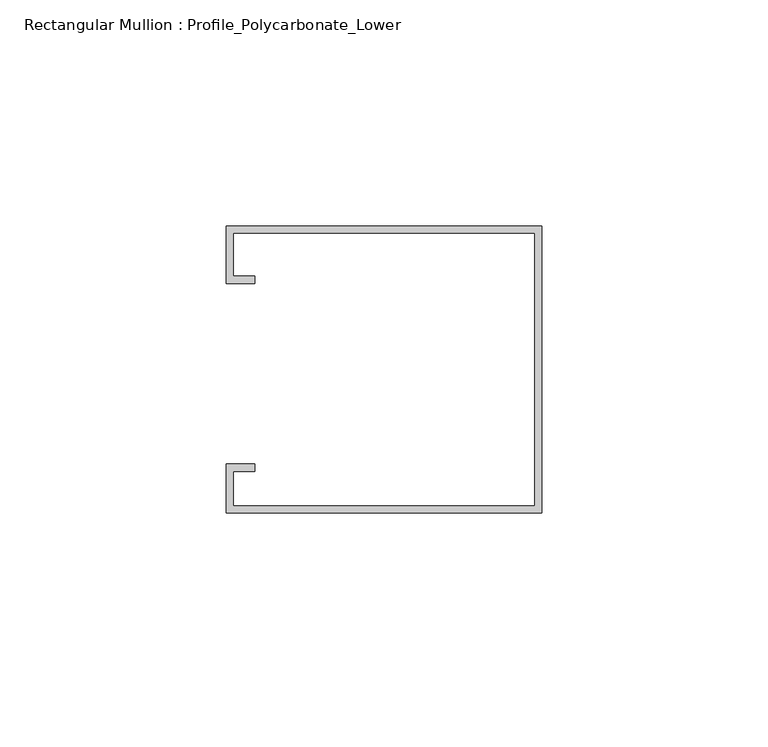
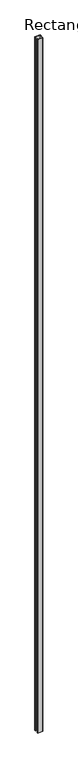
"""IFC4 building model written with IfcOpenShell, lengths in millimetres: member geometry, Rectangular Mullion : Profile_Polycarbonate_Lower."""

from ifc_helpers import new_model, si_unit, frame, origin, place, context, project, spatial, polyline, outline, extrude, source, transform, mapped, element, save


def rectangular_mullion_profile_polycarbonate_lower_4c106b6d(model_context):
    return source(origin(), model_context, "Body", "SweptSolid", [
        extrude(outline(polyline([(0.0, 32.7), (0.0, -30.8), (-69.85, -30.8), (-69.85, -20.0), (-63.5, -20.0), (-63.5, -21.5875), (-68.2625, -21.5875), (-68.2625, -29.2125), (-1.5875, -29.2125), (-1.5875, 31.1125), (-68.2625, 31.1125), (-68.2625, 21.5875), (-63.5, 21.5875), (-63.5, 20.0), (-69.85, 20.0), (-69.85, 32.7), (0.0, 32.7)])), frame((0.0, 0.0, -9907.5875), z_axis=(0.0, 0.0, 1.0), x_axis=(1.0, 0.0, 0.0)), (0.0, 0.0, 1.0), 9907.5875),
    ])


if __name__ == "__main__":
    model = new_model("IFC4")
    model_context = context("Model", 3, world=origin())
    ifc_project = project(units=[si_unit("LENGTHUNIT", "METRE", prefix="MILLI")], contexts=[model_context])
    site = spatial("IfcSite", under=ifc_project)
    building = spatial("IfcBuilding", under=site)
    placement = place(None, origin())
    rectangular_mullion_profile_polycarbonate_lower_shape = rectangular_mullion_profile_polycarbonate_lower_4c106b6d(model_context)
    element("IfcMember", 1, ObjectType="Rectangular Mullion : Profile_Polycarbonate_Lower", at=placement, inside=building, context=model_context, shape_type="MappedRepresentation", body=[
        mapped(rectangular_mullion_profile_polycarbonate_lower_shape, transform((0.0, 0.0, 0.0), x_axis=(1.0, 0.0, 0.0), y_axis=(0.0, 1.0, 0.0), z_axis=(0.0, 0.0, 1.0))),
    ])
    save(model, "model.ifc")

# Revit data of these elements
# Type "Rectangular Mullion : Profile_Polycarbonate_Lower"
#   built-in parameter 1007322 = 0.208333 (stored number, unit not read)
#   built-in parameter 1007321 = 0 (stored number, unit not read)
#   built-in parameter 1007320 = 0.00520833 (stored number, unit not read)
